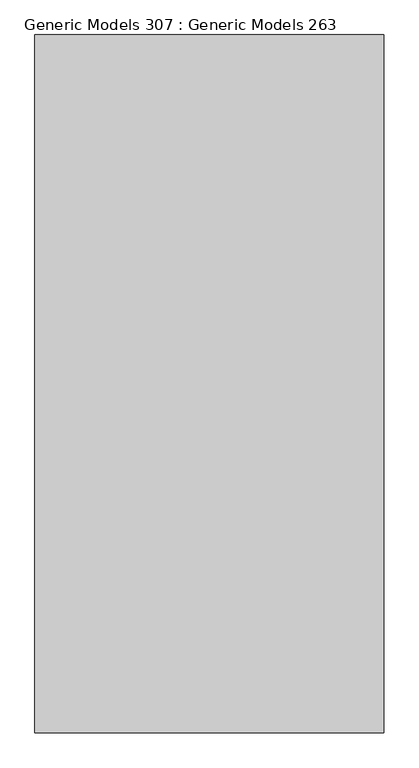
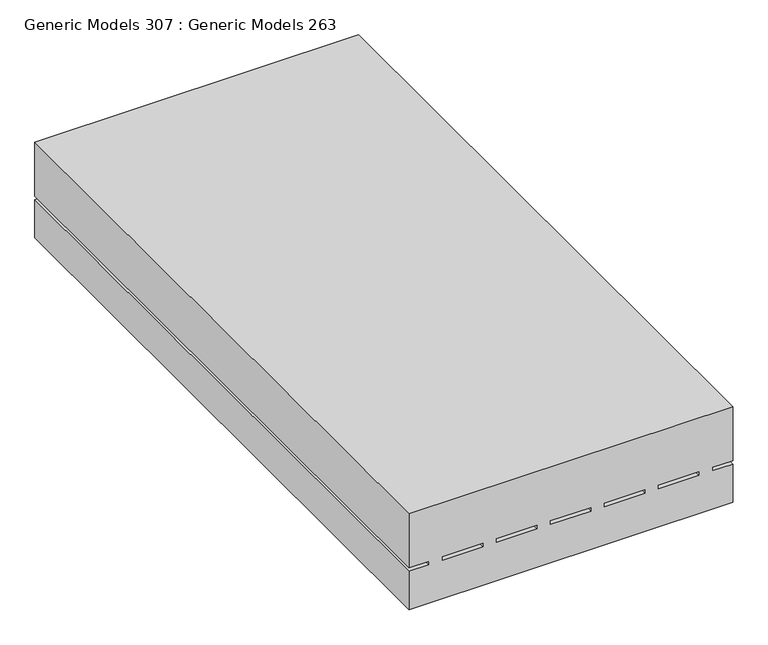
"""IFC4 building model written with IfcOpenShell, lengths in millimetres: proxy geometry, Generic Models 307 : Generic Models 263."""

from ifc_helpers import new_model, si_unit, frame, origin, place, context, project, spatial, polyline, outline, extrude, source, transform, mapped, element, save


def generic_models_307_generic_models_263_524330a5(model_context):
    return source(origin(), model_context, "Body", "SweptSolid", [
        extrude(outline(polyline([(0.0, 95516.9797726), (0.0, 94907.3797726), (-107.2982847, 94907.3797726), (-107.2982847, 94945.4797726), (-114.3, 94945.4797726), (-114.3, 94907.3797726), (-190.5, 94907.3797726), (-190.5, 95516.9797726), (-114.3, 95516.9797726), (-114.3, 95478.8797726), (-107.2982847, 95478.8797726), (-107.2982847, 95516.9797726), (0.0, 95516.9797726)]), holes=[polyline([(-107.2982847, 94970.8797726), (-107.2982847, 95047.0797726), (-114.3, 95047.0797726), (-114.3, 94970.8797726), (-107.2982847, 94970.8797726)]), polyline([(-107.2982847, 95072.4797726), (-107.2982847, 95148.6797726), (-114.3, 95148.6797726), (-114.3, 95072.4797726), (-107.2982847, 95072.4797726)]), polyline([(-107.2982847, 95174.0797726), (-107.2982847, 95250.2797726), (-114.3, 95250.2797726), (-114.3, 95174.0797726), (-107.2982847, 95174.0797726)]), polyline([(-107.2982847, 95275.6797726), (-107.2982847, 95351.8797726), (-114.3, 95351.8797726), (-114.3, 95275.6797726), (-107.2982847, 95275.6797726)]), polyline([(-107.2982847, 95377.2797726), (-107.2982847, 95453.4797726), (-114.3, 95453.4797726), (-114.3, 95377.2797726), (-107.2982847, 95377.2797726)])]), frame((0.0, -94.4486541, 0.0), z_axis=(0.0, 1.0, 0.0), x_axis=(0.0, 0.0, 1.0)), (0.0, 0.0, 1.0), 1219.2),
    ])


if __name__ == "__main__":
    model = new_model("IFC4")
    model_context = context("Model", 3, world=origin())
    ifc_project = project(units=[si_unit("LENGTHUNIT", "METRE", prefix="MILLI")], contexts=[model_context])
    site = spatial("IfcSite", under=ifc_project)
    building = spatial("IfcBuilding", under=site)
    placement = place(None, origin())
    generic_models_307_generic_models_263_shape = generic_models_307_generic_models_263_524330a5(model_context)
    element("IfcBuildingElementProxy", 1, Name="Generic Models 307 : Generic Models 263", ObjectType="Generic Models 307 : Generic Models 263", at=placement, inside=building, context=model_context, shape_type="MappedRepresentation", body=[
        mapped(generic_models_307_generic_models_263_shape, transform((0.0, 0.0, 0.0), x_axis=(1.0, 0.0, 0.0), y_axis=(0.0, 1.0, 0.0), z_axis=(0.0, 0.0, 1.0))),
    ])
    save(model, "model.ifc")

# Revit data of these elements
# Element 1 (IfcBuildingElementProxy, "Generic Models 307 : Generic Models 263")
#   Materials on its faces: "CONCRETE PAVEMENT HEAVY DUTY"
# Materials
#   "CONCRETE PAVEMENT HEAVY DUTY": class "Concrete", colour RGB 191 191 191, transparency 0, Description = "Cast-in-place concrete", Cost = 0
